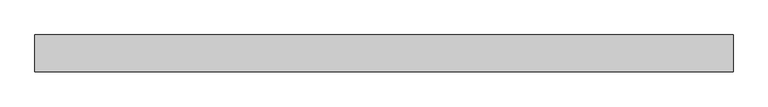
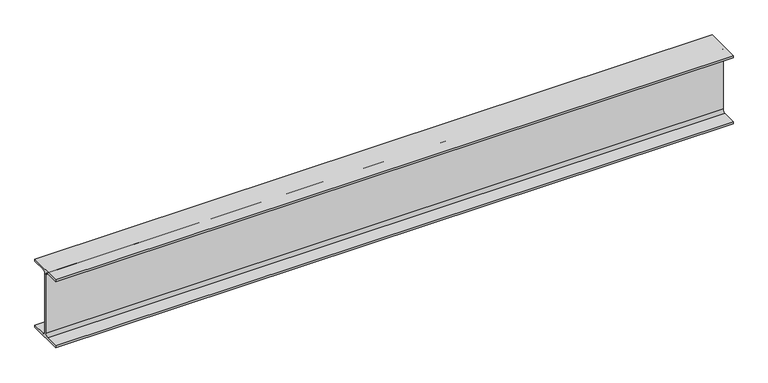
"""IFC4 building model written with IfcOpenShell, lengths in millimetres: beam geometry, Steel Framing_H_KS : H_SB_AR_S02_H-300x150x6.5x9_WG1."""

from ifc_helpers import new_model, si_unit, point, frame, frame_2d, origin, place, context, project, spatial, polyline, circle_curve, trimmed, segment, composite_curve, outline, extrude, source, transform, mapped, element, save


def beam_1a082d06(model_context):
    return source(origin(), model_context, "Body", "SweptSolid", [
        extrude(outline(composite_curve([segment(polyline([(75.0, -141.0), (75.0, -150.0), (-75.0, -150.0), (-75.0, -141.0), (-16.25, -141.0)]), True, "CONTINUOUS"), segment(trimmed(circle_curve(frame_2d((-16.25, -128.0)), 13.0), [point((-16.25, -141.0))], [point((-3.25, -128.0))], True, "CARTESIAN"), True, "CONTINUOUS"), segment(polyline([(-3.25, -128.0), (-3.25, 128.0)]), True, "CONTINUOUS"), segment(trimmed(circle_curve(frame_2d((-16.25, 128.0)), 13.0), [point((-3.25, 128.0))], [point((-16.25, 141.0))], True, "CARTESIAN"), True, "CONTINUOUS"), segment(polyline([(-16.25, 141.0), (-75.0, 141.0), (-75.0, 150.0), (75.0, 150.0), (75.0, 141.0), (16.25, 141.0)]), True, "CONTINUOUS"), segment(trimmed(circle_curve(frame_2d((16.25, 128.0)), 13.0), [point((16.25, 141.0))], [point((3.25, 128.0))], True, "CARTESIAN"), True, "CONTINUOUS"), segment(polyline([(3.25, 128.0), (3.25, -128.0)]), True, "CONTINUOUS"), segment(trimmed(circle_curve(frame_2d((16.25, -128.0)), 13.0), [point((3.25, -128.0))], [point((16.25, -141.0))], True, "CARTESIAN"), True, "CONTINUOUS"), segment(polyline([(16.25, -141.0), (75.0, -141.0)]), True, "CONTINUOUS")], self_intersect=False)), frame((-1412.3, 0.0, 0.0), z_axis=(1.0, 0.0, 0.0), x_axis=(0.0, 1.0, 0.0)), (0.0, 0.0, 1.0), 2824.6),
    ])


if __name__ == "__main__":
    model = new_model("IFC4")
    model_context = context("Model", 3, world=origin())
    ifc_project = project(units=[si_unit("LENGTHUNIT", "METRE", prefix="MILLI")], contexts=[model_context])
    site = spatial("IfcSite", under=ifc_project)
    building = spatial("IfcBuilding", under=site)
    placement = place(None, origin())
    beam_shape = beam_1a082d06(model_context)
    element("IfcBeam", 1, ObjectType="Steel Framing_H_KS : H_SB_AR_S02_H-300x150x6.5x9_WG1", at=placement, inside=building, context=model_context, shape_type="MappedRepresentation", body=[
        mapped(beam_shape, transform((0.0, 0.0, 0.0), x_axis=(1.0, 0.0, 0.0), y_axis=(0.0, 1.0, 0.0), z_axis=(0.0, 0.0, 1.0))),
    ])
    save(model, "model.ifc")

# Revit data of these elements
# Type "Steel Framing_H_KS : H_SB_AR_S02_H-300x150x6.5x9_WG1"
#   Type Comments = "MAIN"
#   Type Mark = "WG1"
#   H_SectionID = "H-300x150x6.5x9"
#   H_Ratio for Additional Steel Plate = 0.2
#   Width = 15.0 cm
#   Web Thickness = 0.65 cm
#   Web Fillet = 1.3 cm
#   Warping Constant = 107000.0 cm⁶
#   Torsional Moment of Inertia = 9.9539 cm⁴
#   Section Area = 46.78 cm²
#   Plastic Modulus weak axis = 105.0 cm³
#   Plastic Modulus strong axis = 542.0 cm³
#   Perimeter = 1.17 m²/m
#   Nominal Weight = 36.70 kgf/m
#   Moment of Inertia weak axis = 508.00 cm⁴
#   Moment of Inertia strong axis = 7210.00 cm⁴
#   Height = 30.0 cm
#   Flange Thickness = 0.9 cm
#   Elastic Modulus weak axis = 67.7 cm³
#   Elastic Modulus strong axis = 481.0 cm³
#   Centroid Vertical = 15.0 cm
#   Centroid Horizontal = 7.5 cm
#   Bolt Spacing = 8.89 cm
#   Length [instance default] = 1500 mm
#   Structural Material [instance default] = Steel, 45-345
#   Section Name Key = ""
#   Assembly Code = ""
# Element 1 (IfcBeam, "Steel Framing_H_KS : H_SB_AR_S02_H-300x150x6.5x9_WG1")
#   Materials on its faces: "Steel, 45-345"
# Materials
#   "Steel, 45-345": class "Metal", colour RGB 189 187 185, transparency 0, Description = "Steel 345 MPa", Cost = 0
